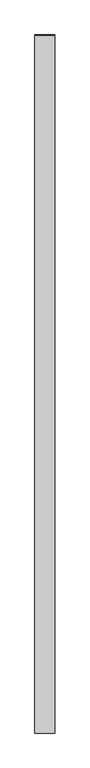
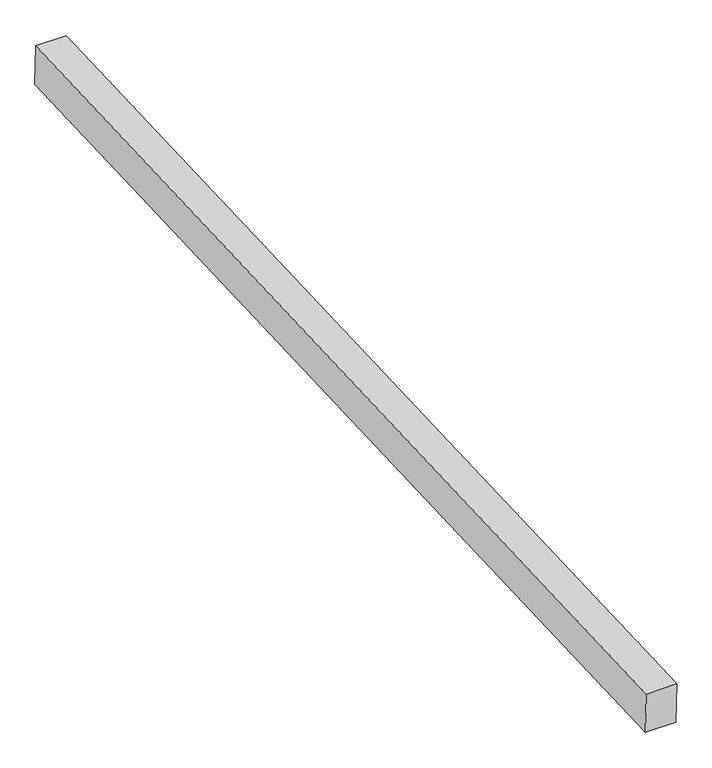
"""IFC4 building model written with IfcOpenShell, lengths in millimetres: proxy geometry, Generic Models 7:Generic Models 1:8:Generic Models 1:8 : Generic Models 7:Generic Models 1:337419:21 : Generic Models 7:Generic Models 1:8:Generic Models 1:8 : Generic Models 7:Generic Models 1:337419:315935."""

from ifc_helpers import new_model, si_unit, frame, origin, place, context, project, spatial, polyline, outline, extrude, source, transform, mapped, element, save


def generic_models_30a192fd(model_context):
    return source(origin(), model_context, "Body", "SweptSolid", [
        extrude(outline(polyline([(-569809.5331551, 8697.9424054), (-564936.6102609, 8900.9808594), (-564929.0433392, 8710.6308549), (-569801.6025364, 8507.607555), (-569809.5331551, 8697.9424054)])), frame((594890.6117243, 0.0, 0.0), z_axis=(1.0, 0.0, 0.0), x_axis=(0.0, 1.0, 0.0)), (0.0, 0.0, 1.0), 139.7),
    ])


if __name__ == "__main__":
    model = new_model("IFC4")
    model_context = context("Model", 3, world=origin())
    ifc_project = project(units=[si_unit("LENGTHUNIT", "METRE", prefix="MILLI")], contexts=[model_context])
    site = spatial("IfcSite", under=ifc_project)
    building = spatial("IfcBuilding", under=site)
    placement = place(None, origin())
    generic_models_shape = generic_models_30a192fd(model_context)
    element("IfcBuildingElementProxy", 1, Name="Generic Models 7:Generic Models 1:8:Generic Models 1:8 : Generic Models 7:Generic Models 1:337419:21 : Generic Models 7:Generic Models 1:8:Generic Models 1:8 : Generic Models 7:Generic Models 1:337419:315935", ObjectType="Generic Models 7:Generic Models 1:8:Generic Models 1:8 : Generic Models 7:Generic Models 1:337419:21 : Generic Models 7:Generic Models 1:8:Generic Models 1:8 : Generic Models 7:Generic Models 1:337419:315935", at=placement, inside=building, context=model_context, shape_type="MappedRepresentation", body=[
        mapped(generic_models_shape, transform((0.0, 0.0, 0.0), x_axis=(1.0, 0.0, 0.0), y_axis=(0.0, 1.0, 0.0), z_axis=(0.0, 0.0, 1.0))),
    ])
    save(model, "model.ifc")

# Revit data of these elements
# Type "Generic Models 7:Generic Models 1:8:Generic Models 1:8 : Generic Models 7:Generic Models 1:337419:21 : Generic Models 7:Generic Models 1:8:Generic Models 1:8 : Generic Models 7:Generic Models 1:337419:315935"
#   NameOverride = "Generic Models 7:Generic Models 1:8:Generic Models 1:8 : Generic Models 7:Generic Models 1:337419:315935"
#   ObjectTypeOverride = "Generic Models 1:8 : Generic Models 7:Generic Models 1:337419"
#   Reference = "Generic Models 1"
#   Tag = "315935"
# Element 1 (IfcBuildingElementProxy, "Generic Models 7:Generic Models 1:8:Generic Models 1:8 : Generic Models 7:Generic Models 1:337419:21 : Generic Models 7:Generic Models 1:8:Generic Models 1:8 : Generic Models 7:Generic Models 1:337419:315935")
#   Materials on its faces: "5 1/2\" X 7 1/2\" EXTERIOR GRADE GLULAM BEAMS"
# Materials
#   "5 1/2\" X 7 1/2\" EXTERIOR GRADE GLULAM BEAMS": class "Wood", colour RGB 183 134 68, transparency 0, Keynote = "M06181300.01", Description = "Pinus Echinata", Cost = 0
